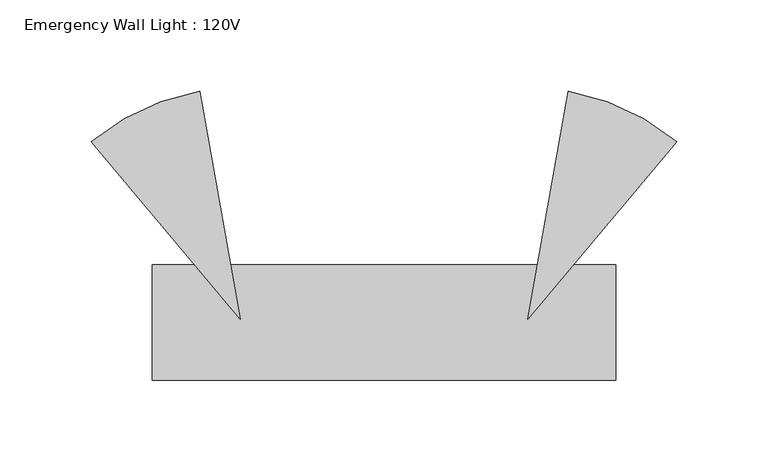
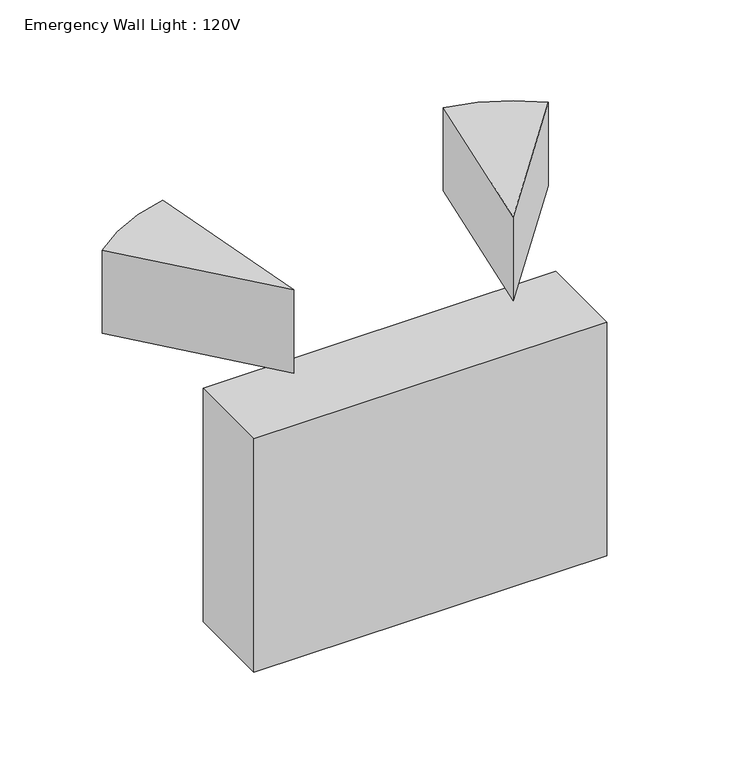
"""IFC4 building model written with IfcOpenShell, lengths in millimetres: light fixture geometry, Emergency Wall Light : 120V."""

import ifcopenshell
import ifcopenshell.guid

model = None  # the IFC model being written
_history = None  # IfcOwnerHistory: only IFC2X3 demands one
_inside = {}  # id of a spatial element -> (the spatial element, [elements in it])
_under = {}  # id of a project, library or spatial element -> (it, [spatial elements below it])
_declared = {}  # id of a project -> (the project, [libraries it declares])
_typed = {}  # id of a type object -> (the type object, [elements of that type])
_made_of = {}  # id of a material, layer set ... -> (it, [elements and type objects made of it])


def new_model(schema):
    """Start an empty IFC model of exactly this schema.

    Asked for "IFC4X3", IfcOpenShell would pick the latest addendum, in which some entities
    have other attributes; the version numbers below select the first issue.
    IFC2X3 requires an IfcOwnerHistory on every rooted entity: one is made here for all.
    """
    global model, _history
    if schema == "IFC4X3":
        model = ifcopenshell.file(schema_version=(4, 3, 0, 0))
    else:
        model = ifcopenshell.file(schema=schema)
    _inside.clear()
    _under.clear()
    _declared.clear()
    _typed.clear()
    _made_of.clear()
    _history = None
    if model.schema == "IFC2X3":
        org = make("IfcOrganization", Name="unknown")
        user = make(
            "IfcPersonAndOrganization",
            ThePerson=make("IfcPerson", FamilyName="unknown"),
            TheOrganization=org,
        )
        app = make(
            "IfcApplication",
            ApplicationDeveloper=org,
            Version="unknown",
            ApplicationFullName="unknown",
            ApplicationIdentifier="unknown",
        )
        _history = make(
            "IfcOwnerHistory",
            OwningUser=user,
            OwningApplication=app,
            ChangeAction="ADDED",
            CreationDate=0,
        )
    return model


def make(cls, **values):
    """One entity of the class cls with the attributes given. An attribute that is None is left unset."""
    return model.create_entity(
        cls, **{name: value for name, value in values.items() if value is not None}
    )


def rooted(cls, **values):
    """An entity with a GlobalId (a new one), such as an element, a storey or a relation."""
    return make(cls, GlobalId=ifcopenshell.guid.new(), OwnerHistory=_history, **values)


def si_unit(unit_type, name, prefix=None):
    """IfcSIUnit, for example si_unit("LENGTHUNIT", "METRE", prefix="MILLI")."""
    return make("IfcSIUnit", UnitType=unit_type, Prefix=prefix, Name=name)


def assignment(units):
    """IfcUnitAssignment: the units of a project."""
    return None if units is None else make("IfcUnitAssignment", Units=units)


def point(xyz):
    """IfcCartesianPoint."""
    return None if xyz is None else make("IfcCartesianPoint", Coordinates=xyz)


def direction(xyz):
    """IfcDirection."""
    return None if xyz is None else make("IfcDirection", DirectionRatios=xyz)


def frame(location, z_axis=None, x_axis=None):
    """IfcAxis2Placement3D, a coordinate frame: its origin and axes. An axis left out is left unset."""
    return make(
        "IfcAxis2Placement3D",
        Location=point(location),
        Axis=direction(z_axis),
        RefDirection=direction(x_axis),
    )


def frame_2d(location, x_axis=None):
    """IfcAxis2Placement2D, a coordinate frame in the plane: its origin and x axis."""
    return make(
        "IfcAxis2Placement2D", Location=point(location), RefDirection=direction(x_axis)
    )


def origin():
    """The frame at (0, 0, 0) with its axes left unset."""
    return frame((0.0, 0.0, 0.0))


def place(relative_to, where):
    """IfcLocalPlacement: puts the frame where relative to a parent placement (None: the world)."""
    return make(
        "IfcLocalPlacement", PlacementRelTo=relative_to, RelativePlacement=where
    )


def context(
    kind, dimensions, precision=None, world=None, true_north=None, identifier=None
):
    """IfcGeometricRepresentationContext, for example the 3D "Model" context."""
    return make(
        "IfcGeometricRepresentationContext",
        ContextIdentifier=identifier,
        ContextType=kind,
        CoordinateSpaceDimension=dimensions,
        Precision=precision,
        WorldCoordinateSystem=world,
        TrueNorth=true_north,
    )


def project(units=None, contexts=None):
    """IfcProject with its units and contexts."""
    return rooted(
        "IfcProject",
        Name="project",
        RepresentationContexts=contexts,
        UnitsInContext=assignment(units),
    )


def spatial(cls, under=None, at=None, **own):
    """A site, building, storey or space (cls), placed at a placement, below another one or the project."""
    s = rooted(cls, ObjectPlacement=at, **own)
    if under is not None:
        _under.setdefault(under.id(), (under, []))[1].append(s)
    return s


def polyline(points):
    """IfcPolyline through the points."""
    return make("IfcPolyline", Points=[point(p) for p in points])


def circle_curve(where, radius):
    """IfcCircle in the frame where."""
    return make("IfcCircle", Position=where, Radius=radius)


def trimmed(basis, trim1, trim2, sense, master):
    """IfcTrimmedCurve: the piece of a basis curve between two trims."""
    return make(
        "IfcTrimmedCurve",
        BasisCurve=basis,
        Trim1=trim1,
        Trim2=trim2,
        SenseAgreement=sense,
        MasterRepresentation=master,
    )


def segment(curve, same_sense, transition):
    """IfcCompositeCurveSegment."""
    return make(
        "IfcCompositeCurveSegment",
        Transition=transition,
        SameSense=same_sense,
        ParentCurve=curve,
    )


def composite_curve(segments, self_intersect=None):
    """IfcCompositeCurve: segments joined end to end."""
    return make("IfcCompositeCurve", Segments=segments, SelfIntersect=self_intersect)


def outline(outer, holes=None, kind="AREA"):
    """IfcArbitraryClosedProfileDef: a profile drawn as a closed curve; with holes, ...WithVoids."""
    if holes is None:
        return make("IfcArbitraryClosedProfileDef", ProfileType=kind, OuterCurve=outer)
    return make(
        "IfcArbitraryProfileDefWithVoids",
        ProfileType=kind,
        OuterCurve=outer,
        InnerCurves=holes,
    )


def extrude(swept, where, along, depth):
    """IfcExtrudedAreaSolid: the profile swept, set in the frame where, extruded along a direction by depth."""
    return make(
        "IfcExtrudedAreaSolid",
        SweptArea=swept,
        Position=where,
        ExtrudedDirection=direction(along),
        Depth=depth,
    )


def shape(context_of_items, identifier, shape_type, items):
    """IfcShapeRepresentation: the items that make up one representation, for example the "Body"."""
    return make(
        "IfcShapeRepresentation",
        ContextOfItems=context_of_items,
        RepresentationIdentifier=identifier,
        RepresentationType=shape_type,
        Items=items,
    )


def source(mapping_origin, context_of_items, identifier, shape_type, items):
    """IfcRepresentationMap: a shape defined once, which mapped items show again and again."""
    return make(
        "IfcRepresentationMap",
        MappingOrigin=mapping_origin,
        MappedRepresentation=shape(context_of_items, identifier, shape_type, items),
    )


def transform(
    local_origin,
    x_axis=None,
    y_axis=None,
    z_axis=None,
    scale=None,
    scale2=None,
    scale3=None,
    uniform=True,
):
    """IfcCartesianTransformationOperator3D, or its non-uniform kind. x_axis, y_axis, z_axis: its Axis1, 2, 3."""
    if uniform:
        return make(
            "IfcCartesianTransformationOperator3D",
            Axis1=direction(x_axis),
            Axis2=direction(y_axis),
            LocalOrigin=point(local_origin),
            Scale=scale,
            Axis3=direction(z_axis),
        )
    return make(
        "IfcCartesianTransformationOperator3DnonUniform",
        Axis1=direction(x_axis),
        Axis2=direction(y_axis),
        LocalOrigin=point(local_origin),
        Scale=scale,
        Axis3=direction(z_axis),
        Scale2=scale2,
        Scale3=scale3,
    )


def mapped(mapping_source, mapping_target):
    """IfcMappedItem: shows the shape of a source again, moved by a transform."""
    return make(
        "IfcMappedItem", MappingSource=mapping_source, MappingTarget=mapping_target
    )


def made_of(thing, what):
    """Note that an element or type object is made of a material, layer set ...; save() writes the relation."""
    if what is not None:
        _made_of.setdefault(what.id(), (what, []))[1].append(thing)
    return thing


def element(
    cls,
    number,
    at=None,
    inside=None,
    cuts=None,
    type_object=None,
    material=None,
    context=None,
    identifier="Body",
    shape_type=None,
    held_by="IfcProductDefinitionShape",
    body=None,
    shapes=None,
    **own,
):
    """One element of the class cls, such as IfcWall. Its Tag is "e" and its number.

    at: its placement. inside: the storey or other place that contains it. cuts: it is an
    opening in that element (IfcRelVoidsElement). A single representation is given by context,
    identifier, shape_type and body (its items); several are given by shapes. held_by: the class
    of the entity that holds the representations. save() writes the other relations.
    """
    e = rooted(cls, Tag="e%d" % number, ObjectPlacement=at, **own)
    if body is not None:
        shapes = [shape(context, identifier, shape_type, body)]
    if shapes is not None:
        e.Representation = make(held_by, Representations=shapes)
    if inside is not None:
        _inside.setdefault(inside.id(), (inside, []))[1].append(e)
    if cuts is not None:
        rooted(
            "IfcRelVoidsElement", RelatingBuildingElement=cuts, RelatedOpeningElement=e
        )
    if type_object is not None:
        _typed.setdefault(type_object.id(), (type_object, []))[1].append(e)
    return made_of(e, material)


def aggregate(whole, parts):
    """IfcRelAggregates: a whole, such as a stair, and the parts it consists of."""
    return rooted("IfcRelAggregates", RelatingObject=whole, RelatedObjects=parts)


def save(model, path):
    """Write the relations noted so far, then the file.

    IfcRelAggregates (storeys below a building ...), IfcRelContainedInSpatialStructure (elements
    in a storey), IfcRelDefinesByType, IfcRelAssociatesMaterial and IfcRelDeclares: one each for
    every whole, place, type object, material and project.
    """
    for whole, parts in _under.values():
        aggregate(whole, parts)
    for where, things in _inside.values():
        rooted(
            "IfcRelContainedInSpatialStructure",
            RelatedElements=things,
            RelatingStructure=where,
        )
    for kind, things in _typed.values():
        rooted("IfcRelDefinesByType", RelatedObjects=things, RelatingType=kind)
    for what, things in _made_of.values():
        rooted("IfcRelAssociatesMaterial", RelatedObjects=things, RelatingMaterial=what)
    for by, libraries in _declared.values():
        rooted("IfcRelDeclares", RelatingContext=by, RelatedDefinitions=libraries)
    model.write(path)


def emergency_wall_light_120v_c4e7ab17(model_context):
    return source(origin(), model_context, "Body", "SweptSolid", [
        extrude(outline(composite_curve([segment(polyline([(-101.0078234, 249.3352305), (-78.9545048, 124.2646459), (-160.5885313, 221.5522902)]), True, "CONTINUOUS"), segment(trimmed(circle_curve(frame_2d((-78.9545048, 124.2646459)), 127.0), [point((-160.5885313, 221.5522902))], [point((-101.0078234, 249.3352305))], False, "CARTESIAN"), True, "CONTINUOUS")], self_intersect=False)), frame((0.0, 0.0, 2235.2), z_axis=(0.0, 0.0, 1.0), x_axis=(1.0, 0.0, 0.0)), (0.0, 0.0, 1.0), 63.5),
        extrude(outline(composite_curve([segment(polyline([(160.5885313, 221.5522902), (78.9545048, 124.2646459), (101.0078234, 249.3352305)]), True, "CONTINUOUS"), segment(trimmed(circle_curve(frame_2d((78.9545048, 124.2646459)), 127.0), [point((101.0078234, 249.3352305))], [point((160.5885313, 221.5522902))], False, "CARTESIAN"), True, "CONTINUOUS")], self_intersect=False)), frame((0.0, 0.0, 2235.2), z_axis=(0.0, 0.0, 1.0), x_axis=(1.0, 0.0, 0.0)), (0.0, 0.0, 1.0), 63.5),
        extrude(outline(polyline([(-127.0, 154.2760654), (127.0, 154.2760654), (127.0, 90.7760654), (-127.0, 90.7760654), (-127.0, 154.2760654)])), frame((0.0, 0.0, 2044.7), z_axis=(0.0, 0.0, 1.0), x_axis=(1.0, 0.0, 0.0)), (0.0, 0.0, 1.0), 177.8),
    ])


if __name__ == "__main__":
    model = new_model("IFC4")
    model_context = context("Model", 3, world=origin())
    ifc_project = project(units=[si_unit("LENGTHUNIT", "METRE", prefix="MILLI")], contexts=[model_context])
    site = spatial("IfcSite", under=ifc_project)
    building = spatial("IfcBuilding", under=site)
    placement = place(None, origin())
    emergency_wall_light_120v_shape = emergency_wall_light_120v_c4e7ab17(model_context)
    element("IfcLightFixture", 1, ObjectType="Emergency Wall Light : 120V", at=placement, inside=building, context=model_context, shape_type="MappedRepresentation", body=[
        mapped(emergency_wall_light_120v_shape, transform((0.0, 0.0, 0.0), x_axis=(1.0, 0.0, 0.0), y_axis=(0.0, 1.0, 0.0), z_axis=(0.0, 0.0, 1.0))),
    ])
    save(model, "model.ifc")

# Revit data of these elements
# Type "Emergency Wall Light : 120V"
#   Lamp = "A-19"
#   Assembly Code = "D5090200"
#   Wattage Comments = "100"
#   Ballast Voltage = 120 V
#   Mounting Height = 7' - 0"
#   Apparent Load = 100 VA
#   Ballast Number of Poles = 1
#   Load Classification = Lighting - Dwelling Unit
#   Light Casing = Steel, Paint Finish, Ivory, Glossy
# Element 1 (IfcLightFixture, "Emergency Wall Light : 120V")
#   Materials on its faces: "Steel, Paint Finish, Ivory, Glossy"
# Materials
#   "Steel, Paint Finish, Ivory, Glossy": class "Metal", colour RGB 247 247 239, transparency 0, Description = "Steel, paint finish, ivory, glossy", Cost = 0
